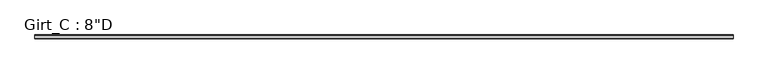
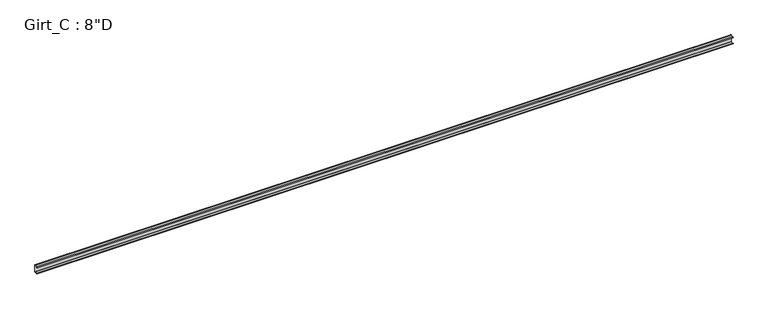
"""IFC4 building model written with IfcOpenShell, lengths in millimetres: beam geometry."""

import ifcopenshell
import ifcopenshell.guid

model = None  # the IFC model being written
_history = None  # IfcOwnerHistory: only IFC2X3 demands one
_inside = {}  # id of a spatial element -> (the spatial element, [elements in it])
_under = {}  # id of a project, library or spatial element -> (it, [spatial elements below it])
_declared = {}  # id of a project -> (the project, [libraries it declares])
_typed = {}  # id of a type object -> (the type object, [elements of that type])
_made_of = {}  # id of a material, layer set ... -> (it, [elements and type objects made of it])


def new_model(schema):
    """Start an empty IFC model of exactly this schema.

    Asked for "IFC4X3", IfcOpenShell would pick the latest addendum, in which some entities
    have other attributes; the version numbers below select the first issue.
    IFC2X3 requires an IfcOwnerHistory on every rooted entity: one is made here for all.
    """
    global model, _history
    if schema == "IFC4X3":
        model = ifcopenshell.file(schema_version=(4, 3, 0, 0))
    else:
        model = ifcopenshell.file(schema=schema)
    _inside.clear()
    _under.clear()
    _declared.clear()
    _typed.clear()
    _made_of.clear()
    _history = None
    if model.schema == "IFC2X3":
        org = make("IfcOrganization", Name="unknown")
        user = make(
            "IfcPersonAndOrganization",
            ThePerson=make("IfcPerson", FamilyName="unknown"),
            TheOrganization=org,
        )
        app = make(
            "IfcApplication",
            ApplicationDeveloper=org,
            Version="unknown",
            ApplicationFullName="unknown",
            ApplicationIdentifier="unknown",
        )
        _history = make(
            "IfcOwnerHistory",
            OwningUser=user,
            OwningApplication=app,
            ChangeAction="ADDED",
            CreationDate=0,
        )
    return model


def make(cls, **values):
    """One entity of the class cls with the attributes given. An attribute that is None is left unset."""
    return model.create_entity(
        cls, **{name: value for name, value in values.items() if value is not None}
    )


def rooted(cls, **values):
    """An entity with a GlobalId (a new one), such as an element, a storey or a relation."""
    return make(cls, GlobalId=ifcopenshell.guid.new(), OwnerHistory=_history, **values)


def si_unit(unit_type, name, prefix=None):
    """IfcSIUnit, for example si_unit("LENGTHUNIT", "METRE", prefix="MILLI")."""
    return make("IfcSIUnit", UnitType=unit_type, Prefix=prefix, Name=name)


def assignment(units):
    """IfcUnitAssignment: the units of a project."""
    return None if units is None else make("IfcUnitAssignment", Units=units)


def point(xyz):
    """IfcCartesianPoint."""
    return None if xyz is None else make("IfcCartesianPoint", Coordinates=xyz)


def direction(xyz):
    """IfcDirection."""
    return None if xyz is None else make("IfcDirection", DirectionRatios=xyz)


def frame(location, z_axis=None, x_axis=None):
    """IfcAxis2Placement3D, a coordinate frame: its origin and axes. An axis left out is left unset."""
    return make(
        "IfcAxis2Placement3D",
        Location=point(location),
        Axis=direction(z_axis),
        RefDirection=direction(x_axis),
    )


def frame_2d(location, x_axis=None):
    """IfcAxis2Placement2D, a coordinate frame in the plane: its origin and x axis."""
    return make(
        "IfcAxis2Placement2D", Location=point(location), RefDirection=direction(x_axis)
    )


def origin():
    """The frame at (0, 0, 0) with its axes left unset."""
    return frame((0.0, 0.0, 0.0))


def place(relative_to, where):
    """IfcLocalPlacement: puts the frame where relative to a parent placement (None: the world)."""
    return make(
        "IfcLocalPlacement", PlacementRelTo=relative_to, RelativePlacement=where
    )


def context(
    kind, dimensions, precision=None, world=None, true_north=None, identifier=None
):
    """IfcGeometricRepresentationContext, for example the 3D "Model" context."""
    return make(
        "IfcGeometricRepresentationContext",
        ContextIdentifier=identifier,
        ContextType=kind,
        CoordinateSpaceDimension=dimensions,
        Precision=precision,
        WorldCoordinateSystem=world,
        TrueNorth=true_north,
    )


def project(units=None, contexts=None):
    """IfcProject with its units and contexts."""
    return rooted(
        "IfcProject",
        Name="project",
        RepresentationContexts=contexts,
        UnitsInContext=assignment(units),
    )


def spatial(cls, under=None, at=None, **own):
    """A site, building, storey or space (cls), placed at a placement, below another one or the project."""
    s = rooted(cls, ObjectPlacement=at, **own)
    if under is not None:
        _under.setdefault(under.id(), (under, []))[1].append(s)
    return s


def polyline(points):
    """IfcPolyline through the points."""
    return make("IfcPolyline", Points=[point(p) for p in points])


def circle_curve(where, radius):
    """IfcCircle in the frame where."""
    return make("IfcCircle", Position=where, Radius=radius)


def trimmed(basis, trim1, trim2, sense, master):
    """IfcTrimmedCurve: the piece of a basis curve between two trims."""
    return make(
        "IfcTrimmedCurve",
        BasisCurve=basis,
        Trim1=trim1,
        Trim2=trim2,
        SenseAgreement=sense,
        MasterRepresentation=master,
    )


def segment(curve, same_sense, transition):
    """IfcCompositeCurveSegment."""
    return make(
        "IfcCompositeCurveSegment",
        Transition=transition,
        SameSense=same_sense,
        ParentCurve=curve,
    )


def composite_curve(segments, self_intersect=None):
    """IfcCompositeCurve: segments joined end to end."""
    return make("IfcCompositeCurve", Segments=segments, SelfIntersect=self_intersect)


def outline(outer, holes=None, kind="AREA"):
    """IfcArbitraryClosedProfileDef: a profile drawn as a closed curve; with holes, ...WithVoids."""
    if holes is None:
        return make("IfcArbitraryClosedProfileDef", ProfileType=kind, OuterCurve=outer)
    return make(
        "IfcArbitraryProfileDefWithVoids",
        ProfileType=kind,
        OuterCurve=outer,
        InnerCurves=holes,
    )


def extrude(swept, where, along, depth):
    """IfcExtrudedAreaSolid: the profile swept, set in the frame where, extruded along a direction by depth."""
    return make(
        "IfcExtrudedAreaSolid",
        SweptArea=swept,
        Position=where,
        ExtrudedDirection=direction(along),
        Depth=depth,
    )


def shape(context_of_items, identifier, shape_type, items):
    """IfcShapeRepresentation: the items that make up one representation, for example the "Body"."""
    return make(
        "IfcShapeRepresentation",
        ContextOfItems=context_of_items,
        RepresentationIdentifier=identifier,
        RepresentationType=shape_type,
        Items=items,
    )


def source(mapping_origin, context_of_items, identifier, shape_type, items):
    """IfcRepresentationMap: a shape defined once, which mapped items show again and again."""
    return make(
        "IfcRepresentationMap",
        MappingOrigin=mapping_origin,
        MappedRepresentation=shape(context_of_items, identifier, shape_type, items),
    )


def transform(
    local_origin,
    x_axis=None,
    y_axis=None,
    z_axis=None,
    scale=None,
    scale2=None,
    scale3=None,
    uniform=True,
):
    """IfcCartesianTransformationOperator3D, or its non-uniform kind. x_axis, y_axis, z_axis: its Axis1, 2, 3."""
    if uniform:
        return make(
            "IfcCartesianTransformationOperator3D",
            Axis1=direction(x_axis),
            Axis2=direction(y_axis),
            LocalOrigin=point(local_origin),
            Scale=scale,
            Axis3=direction(z_axis),
        )
    return make(
        "IfcCartesianTransformationOperator3DnonUniform",
        Axis1=direction(x_axis),
        Axis2=direction(y_axis),
        LocalOrigin=point(local_origin),
        Scale=scale,
        Axis3=direction(z_axis),
        Scale2=scale2,
        Scale3=scale3,
    )


def mapped(mapping_source, mapping_target):
    """IfcMappedItem: shows the shape of a source again, moved by a transform."""
    return make(
        "IfcMappedItem", MappingSource=mapping_source, MappingTarget=mapping_target
    )


def made_of(thing, what):
    """Note that an element or type object is made of a material, layer set ...; save() writes the relation."""
    if what is not None:
        _made_of.setdefault(what.id(), (what, []))[1].append(thing)
    return thing


def element(
    cls,
    number,
    at=None,
    inside=None,
    cuts=None,
    type_object=None,
    material=None,
    context=None,
    identifier="Body",
    shape_type=None,
    held_by="IfcProductDefinitionShape",
    body=None,
    shapes=None,
    **own,
):
    """One element of the class cls, such as IfcWall. Its Tag is "e" and its number.

    at: its placement. inside: the storey or other place that contains it. cuts: it is an
    opening in that element (IfcRelVoidsElement). A single representation is given by context,
    identifier, shape_type and body (its items); several are given by shapes. held_by: the class
    of the entity that holds the representations. save() writes the other relations.
    """
    e = rooted(cls, Tag="e%d" % number, ObjectPlacement=at, **own)
    if body is not None:
        shapes = [shape(context, identifier, shape_type, body)]
    if shapes is not None:
        e.Representation = make(held_by, Representations=shapes)
    if inside is not None:
        _inside.setdefault(inside.id(), (inside, []))[1].append(e)
    if cuts is not None:
        rooted(
            "IfcRelVoidsElement", RelatingBuildingElement=cuts, RelatedOpeningElement=e
        )
    if type_object is not None:
        _typed.setdefault(type_object.id(), (type_object, []))[1].append(e)
    return made_of(e, material)


def aggregate(whole, parts):
    """IfcRelAggregates: a whole, such as a stair, and the parts it consists of."""
    return rooted("IfcRelAggregates", RelatingObject=whole, RelatedObjects=parts)


def save(model, path):
    """Write the relations noted so far, then the file.

    IfcRelAggregates (storeys below a building ...), IfcRelContainedInSpatialStructure (elements
    in a storey), IfcRelDefinesByType, IfcRelAssociatesMaterial and IfcRelDeclares: one each for
    every whole, place, type object, material and project.
    """
    for whole, parts in _under.values():
        aggregate(whole, parts)
    for where, things in _inside.values():
        rooted(
            "IfcRelContainedInSpatialStructure",
            RelatedElements=things,
            RelatingStructure=where,
        )
    for kind, things in _typed.values():
        rooted("IfcRelDefinesByType", RelatedObjects=things, RelatingType=kind)
    for what, things in _made_of.values():
        rooted("IfcRelAssociatesMaterial", RelatedObjects=things, RelatingMaterial=what)
    for by, libraries in _declared.values():
        rooted("IfcRelDeclares", RelatingContext=by, RelatedDefinitions=libraries)
    model.write(path)


def beam_9edf529d(model_context):
    return source(origin(), model_context, "Body", "SweptSolid", [
        extrude(outline(composite_curve([segment(polyline([(-87.5109375, 101.6), (-3.3734375, 101.6)]), True, "CONTINUOUS"), segment(trimmed(circle_curve(frame_2d((-3.3734375, 96.8375)), 4.7625), [point((-3.3734375, 101.6))], [point((1.3890625, 96.8375))], False, "CARTESIAN"), True, "CONTINUOUS"), segment(polyline([(1.3890625, 96.8375), (1.3890625, -96.8375)]), True, "CONTINUOUS"), segment(trimmed(circle_curve(frame_2d((-3.3734375, -96.8375)), 4.7625), [point((1.3890625, -96.8375))], [point((-3.3734375, -101.6))], False, "CARTESIAN"), True, "CONTINUOUS"), segment(polyline([(-3.3734375, -101.6), (-87.5109375, -101.6), (-99.7792647, -86.979177), (-97.6510975, -85.1934327), (-86.2154765, -98.821875), (-3.2694106, -98.821875)]), True, "CONTINUOUS"), segment(trimmed(circle_curve(frame_2d((-3.3748024, -96.8389339)), 1.9857399), [point((-3.2694106, -98.821875))], [point((-1.3890625, -96.8389339))], True, "CARTESIAN"), True, "CONTINUOUS"), segment(polyline([(-1.3890625, -96.8389339), (-1.3890625, 96.8381931)]), True, "CONTINUOUS"), segment(trimmed(circle_curve(frame_2d((-3.3741066, 96.8381931)), 1.9850441), [point((-1.3890625, 96.8381931))], [point((-3.3005807, 98.821875))], True, "CARTESIAN"), True, "CONTINUOUS"), segment(polyline([(-3.3005807, 98.821875), (-86.2154765, 98.821875), (-97.6278742, 85.221109), (-99.7560415, 87.0068534), (-87.5109375, 101.6)]), True, "CONTINUOUS")], self_intersect=False)), frame((-9256.8059343, 0.0, 0.0), z_axis=(1.0, 0.0, 0.0), x_axis=(0.0, 1.0, 0.0)), (0.0, 0.0, 1.0), 19092.545),
    ])


if __name__ == "__main__":
    model = new_model("IFC4")
    model_context = context("Model", 3, world=origin())
    ifc_project = project(units=[si_unit("LENGTHUNIT", "METRE", prefix="MILLI")], contexts=[model_context])
    site = spatial("IfcSite", under=ifc_project)
    building = spatial("IfcBuilding", under=site)
    placement = place(None, origin())
    beam_shape = beam_9edf529d(model_context)
    element("IfcBeam", 1, ObjectType="Girt_C : 8\"D", at=placement, inside=building, context=model_context, shape_type="MappedRepresentation", body=[
        mapped(beam_shape, transform((0.0, 0.0, 0.0), x_axis=(1.0, 0.0, 0.0), y_axis=(0.0, 1.0, 0.0), z_axis=(0.0, 0.0, 1.0))),
    ])
    save(model, "model.ifc")

# Revit data of these elements
# Type "Girt_C : 8\"D"
#   half leg = 0' - 1 3/4"
#   Web_Thickness = 0' - 0 7/64"
#   Length [instance default] = 10' - 0"
#   Leg_1 = 0' - 3 1/2"
#   Height = 0' - 8"
#   Structural Material [instance default] = none
# Element 1 (IfcBeam, "Girt_C : 8\"D")
#   Structural Material = CEE' SECTION (8.0x3.5C - SEE STRUCT. DWGS)
#   Materials on its faces: "CEE' SECTION (8.0x3.5C - SEE STRUCT. DWGS)"
# Materials
#   "CEE' SECTION (8.0x3.5C - SEE STRUCT. DWGS)": class "Metal", colour RGB 137 146 153, transparency 0, Description = "Steel, mill finish", Cost = 0
